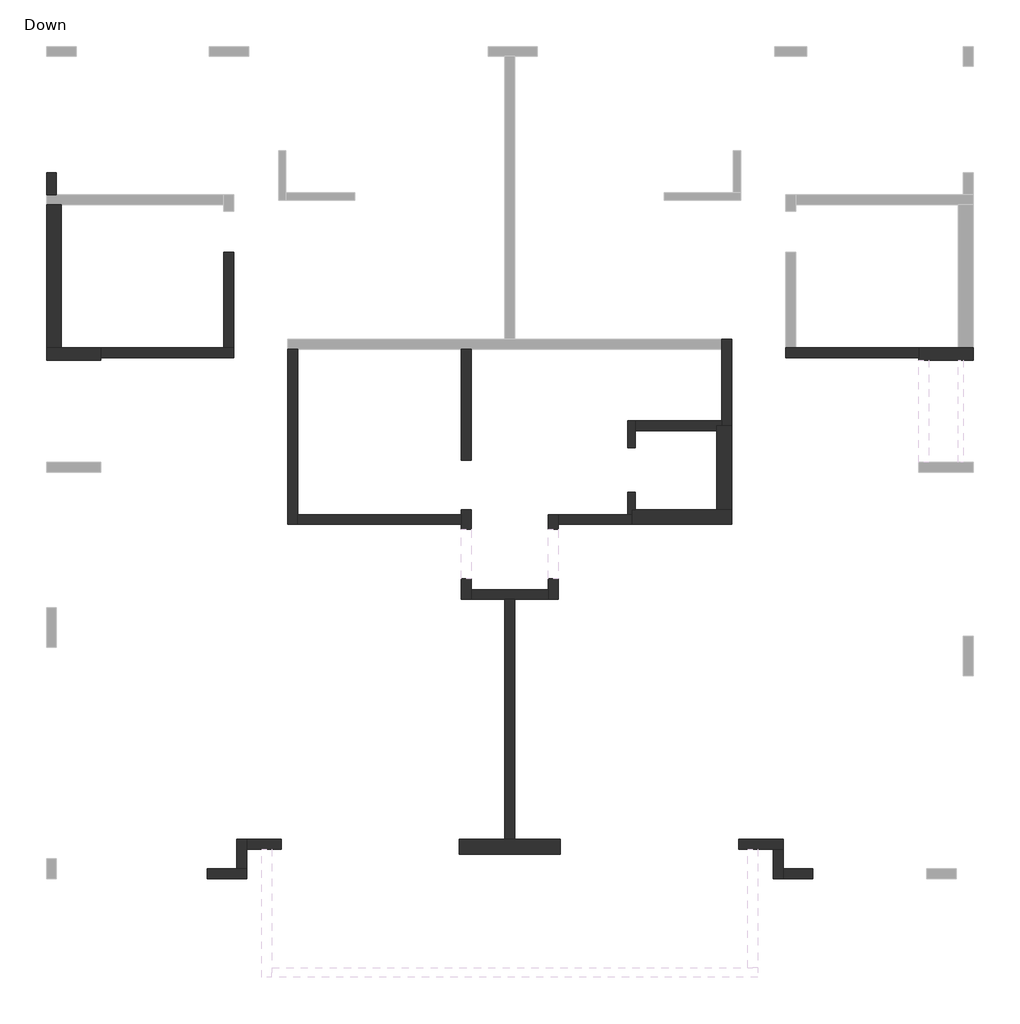
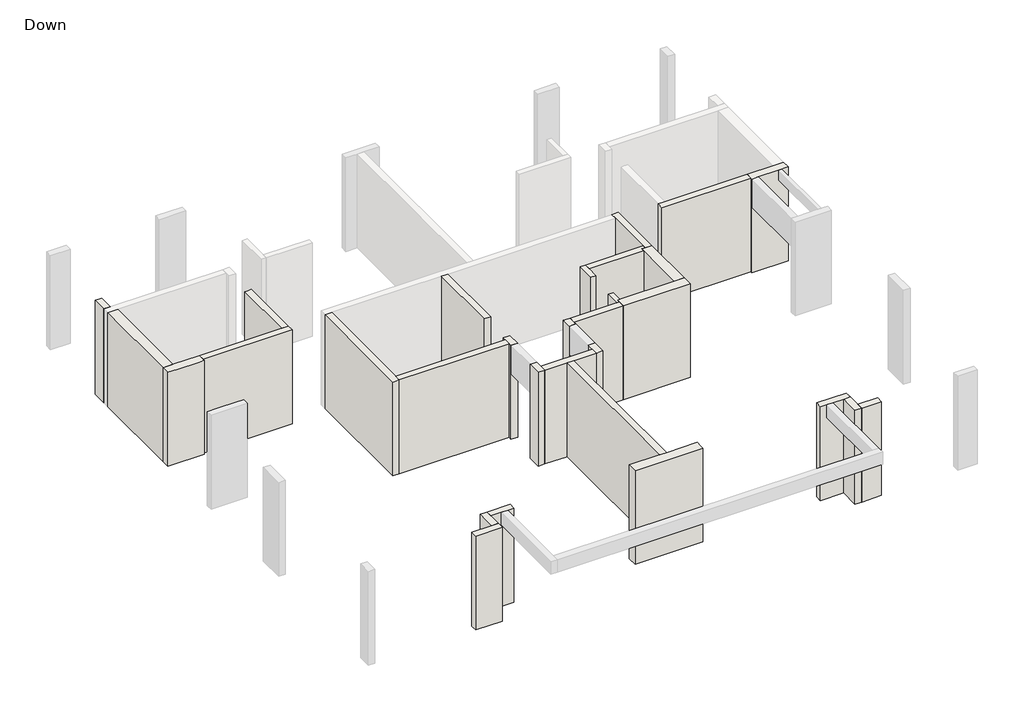
# One storey, part 1 of 2: 30 walls.
"""IFC4 building model written with IfcOpenShell, lengths in millimetres."""

from ifc_helpers import new_model, si_unit, origin, place, context, project, spatial, faceted_brep, element, save

model = new_model("IFC4")

# Units and contexts
model_context = context("Model", 3, world=origin())
ifc_project = project(units=[si_unit("LENGTHUNIT", "METRE", prefix="MILLI")], contexts=[model_context])

# Site, building, storey
site = spatial("IfcSite", under=ifc_project)
building = spatial("IfcBuilding", under=site)
storey = spatial("IfcBuildingStorey", under=building, Name="Down", Elevation=0.0)

# Walls
placement = place(None, origin())
element("IfcWall", 1, ObjectType="15", at=placement, inside=storey, context=model_context, shape_type="Brep", body=[
    faceted_brep([(-36032.8992549, 30554.4375606, 0.0), (-36032.8992549, 30005.16433, 0.0), (-36032.8992549, 30005.16433, 2780.0), (-36032.8992549, 30005.16433, 3000.0), (-36032.8992549, 30554.4375606, 3000.0), (-36032.8992549, 30554.4375606, 2780.0), (-35882.8992549, 30554.4375606, 0.0), (-35882.8992549, 30554.4375606, 3000.0), (-35882.8992549, 30354.4375606, 3000.0), (-35882.8992549, 30005.16433, 3000.0), (-35882.8992549, 30005.16433, 2780.0), (-35882.8992549, 30005.16433, 0.0), (-35882.8992549, 30354.4375606, 0.0)], [[[0, 1, 2, 3, 4, 5]], [[6, 7, 8, 9, 10, 11, 12]], [[1, 0, 6, 12, 11]], [[3, 2, 1, 11, 10, 9]], [[4, 3, 9, 8, 7]], [[0, 5, 4, 7, 6]]]),
])
element("IfcWall", 2, ObjectType="15", at=placement, inside=storey, context=model_context, shape_type="Brep", body=[
    faceted_brep([(-36032.8992549, 29103.4696053, 0.0), (-36032.8992549, 28654.7268324, 0.0), (-36032.8992549, 28654.7268324, 2780.0), (-36032.8992549, 28654.7268324, 3000.0), (-36032.8992549, 29103.4696053, 3000.0), (-36032.8992549, 29103.4696053, 2780.0), (-35882.8992549, 29103.4696053, 0.0), (-35882.8992549, 29103.4696053, 2780.0), (-35882.8992549, 29103.4696053, 3000.0), (-35882.8992549, 28754.7268324, 3000.0), (-35882.8992549, 28754.7268324, 0.0), (-35957.8992549, 28754.7268324, 0.0), (-35957.8992549, 28654.7268324, 0.0), (-35957.8992549, 28654.7268324, 3000.0), (-35957.8992549, 28754.7268324, 3000.0)], [[[0, 1, 2, 3, 4, 5]], [[6, 7, 8, 9, 10]], [[1, 0, 6, 10, 11, 12]], [[4, 3, 13, 14, 9, 8]], [[0, 5, 4, 8, 7, 6]], [[3, 2, 1, 12, 13]], [[12, 11, 14, 13]], [[11, 10, 9, 14]]]),
])
element("IfcWall", 3, ObjectType="20", at=placement, inside=storey, context=model_context, shape_type="Brep", body=[
    faceted_brep([(-38324.2014504, 22079.8085502, 0.0), (-38324.2014504, 26934.5299537, 0.0), (-38324.2014504, 26934.5299537, 2780.0), (-38324.2014504, 26934.5299537, 3000.0), (-38324.2014504, 22079.8085502, 3000.0), (-38324.2014504, 22079.8085502, 2780.0), (-38524.2014504, 22079.8085502, 0.0), (-38524.2014504, 22079.8085502, 2780.0), (-38524.2014504, 22079.8085502, 3000.0), (-38524.2014504, 26934.5299537, 3000.0), (-38524.2014504, 26934.5299537, 2780.0), (-38524.2014504, 26934.5299537, 0.0)], [[[0, 1, 2, 3, 4, 5]], [[6, 7, 8, 9, 10, 11]], [[1, 0, 6, 11]], [[4, 3, 9, 8]], [[3, 2, 1, 11, 10, 9]], [[0, 5, 4, 8, 7, 6]]]),
])
element("IfcWall", 4, ObjectType="20", at=placement, inside=storey, context=model_context, shape_type="Brep", body=[
    faceted_brep([(-39204.7173594, 26934.5299537, 0.0), (-38524.2014504, 26934.5299537, 0.0), (-38324.2014504, 26934.5299537, 0.0), (-37644.7021495, 26934.5299537, 0.0), (-37644.7021495, 26934.5299537, 3000.0), (-38324.2014504, 26934.5299537, 3000.0), (-38524.2014504, 26934.5299537, 3000.0), (-39204.7173594, 26934.5299537, 3000.0), (-39204.7173594, 27134.5299537, 0.0), (-39204.7173594, 27134.5299537, 2780.0), (-39204.7173594, 27134.5299537, 3000.0), (-37644.7021495, 27134.5299537, 3000.0), (-37644.7021495, 27134.5299537, 2780.0), (-37644.7021495, 27134.5299537, 0.0)], [[[0, 1, 2, 3, 4, 5, 6, 7]], [[8, 9, 10, 11, 12, 13]], [[3, 2, 1, 0, 8, 13]], [[7, 6, 5, 4, 11, 10]], [[4, 3, 13, 12, 11]], [[0, 7, 10, 9, 8]]]),
])
element("IfcWall", 5, ObjectType="20", at=placement, inside=storey, context=model_context, shape_type="Brep", body=[
    faceted_brep([(-37444.7021495, 26934.5299537, 0.0), (-37444.7021495, 27352.982888, 0.0), (-37444.7021495, 27352.982888, 2100.0), (-37444.7021495, 27352.982888, 3000.0), (-37444.7021495, 26934.5299537, 3000.0), (-37444.7021495, 26934.5299537, 2780.0), (-37644.7021495, 26934.5299537, 0.0), (-37644.7021495, 26934.5299537, 3000.0), (-37644.7021495, 27134.5299537, 3000.0), (-37644.7021495, 27352.982888, 3000.0), (-37644.7021495, 27352.982888, 2100.0), (-37644.7021495, 27352.982888, 0.0), (-37644.7021495, 27134.5299537, 0.0)], [[[0, 1, 2, 3, 4, 5]], [[6, 7, 8, 9, 10, 11, 12]], [[1, 0, 6, 12, 11]], [[3, 2, 1, 11, 10, 9]], [[4, 3, 9, 8, 7]], [[0, 5, 4, 7, 6]]]),
])
element("IfcWall", 6, ObjectType="20", at=placement, inside=storey, context=model_context, shape_type="Brep", body=[
    faceted_brep([(-39204.7173594, 26934.5299537, 0.0), (-39204.7173594, 27134.5299537, 0.0), (-39204.7173594, 27352.982888, 0.0), (-39204.7173594, 27352.982888, 2100.0), (-39204.7173594, 27352.982888, 3000.0), (-39204.7173594, 27134.5299537, 3000.0), (-39204.7173594, 26934.5299537, 3000.0), (-39404.7173594, 26934.5299537, 0.0), (-39404.7173594, 26934.5299537, 2780.0), (-39404.7173594, 26934.5299537, 3000.0), (-39404.7173594, 27352.982888, 3000.0), (-39404.7173594, 27352.982888, 2100.0), (-39404.7173594, 27352.982888, 0.0)], [[[0, 1, 2, 3, 4, 5, 6]], [[7, 8, 9, 10, 11, 12]], [[2, 1, 0, 7, 12]], [[4, 3, 2, 12, 11, 10]], [[6, 5, 4, 10, 9]], [[0, 6, 9, 8, 7]]]),
])
element("IfcWall", 7, ObjectType="20", at=placement, inside=storey, context=model_context, shape_type="Brep", body=[
    faceted_brep([(-37444.7021495, 28354.1914622, 0.0), (-37444.7021495, 28454.7268324, 0.0), (-37444.7021495, 28654.7268324, 0.0), (-37444.7021495, 28654.7268324, 3000.0), (-37444.7021495, 28454.7268324, 3000.0), (-37444.7021495, 28354.1914622, 3000.0), (-37444.7021495, 28354.1914622, 2100.0), (-37644.7021495, 28354.1914622, 0.0), (-37644.7021495, 28354.1914622, 2100.0), (-37644.7021495, 28354.1914622, 3000.0), (-37644.7021495, 28654.7268324, 3000.0), (-37644.7021495, 28654.7268324, 2780.0), (-37644.7021495, 28654.7268324, 0.0)], [[[0, 1, 2, 3, 4, 5, 6]], [[7, 8, 9, 10, 11, 12]], [[2, 1, 0, 7, 12]], [[5, 4, 3, 10, 9]], [[0, 6, 5, 9, 8, 7]], [[3, 2, 12, 11, 10]]]),
])
element("IfcWall", 8, ObjectType="20", at=placement, inside=storey, context=model_context, shape_type="Brep", body=[
    faceted_brep([(-37444.7021495, 28454.7268324, 0.0), (-35957.8992549, 28454.7268324, 0.0), (-35957.8992549, 28454.7268324, 3000.0), (-37444.7021495, 28454.7268324, 3000.0), (-37444.7021495, 28454.7268324, 2780.0), (-37444.7021495, 28654.7268324, 0.0), (-37444.7021495, 28654.7268324, 3000.0), (-36032.8992549, 28654.7268324, 3000.0), (-35957.8992549, 28654.7268324, 3000.0), (-35957.8992549, 28654.7268324, 0.0), (-36032.8992549, 28654.7268324, 0.0)], [[[0, 1, 2, 3, 4]], [[5, 6, 7, 8, 9, 10]], [[1, 0, 5, 10, 9]], [[2, 1, 9, 8]], [[3, 2, 8, 7, 6]], [[0, 4, 3, 6, 5]]]),
])
element("IfcWall", 9, ObjectType="20", at=placement, inside=storey, context=model_context, shape_type="Brep", body=[
    faceted_brep([(-33933.139307, 30454.4375606, 0.0), (-33933.139307, 32204.3938202, 0.0), (-33933.139307, 32204.3938202, 2780.0), (-33933.139307, 32204.3938202, 3000.0), (-33933.139307, 30454.4375606, 3000.0), (-34133.139307, 30454.4375606, 0.0), (-34133.139307, 30454.4375606, 3000.0), (-34133.139307, 30554.4375606, 3000.0), (-34133.139307, 32004.3938202, 3000.0), (-34133.139307, 32204.3938202, 3000.0), (-34133.139307, 32204.3938202, 0.0), (-34133.139307, 32004.3938202, 0.0), (-34133.139307, 30554.4375606, 0.0)], [[[0, 1, 2, 3, 4]], [[5, 6, 7, 8, 9, 10, 11, 12]], [[1, 0, 5, 12, 11, 10]], [[4, 3, 9, 8, 7, 6]], [[0, 4, 6, 5]], [[3, 2, 1, 10, 9]]]),
])
element("IfcWall", 10, ObjectType="20", at=placement, inside=storey, context=model_context, shape_type="Brep", body=[
    faceted_brep([(-42920.5336878, 32004.3938202, 0.0), (-42920.5336878, 28453.6610046, 0.0), (-42920.5336878, 28453.6610046, 2780.0), (-42920.5336878, 28453.6610046, 3000.0), (-42920.5336878, 32004.3938202, 3000.0), (-42720.5336878, 32004.3938202, 0.0), (-42720.5336878, 32004.3938202, 3000.0), (-42720.5336878, 28653.6610046, 3000.0), (-42720.5336878, 28453.6610046, 3000.0), (-42720.5336878, 28453.6610046, 0.0), (-42720.5336878, 28653.6610046, 0.0)], [[[0, 1, 2, 3, 4]], [[5, 6, 7, 8, 9, 10]], [[1, 0, 5, 10, 9]], [[4, 3, 8, 7, 6]], [[0, 4, 6, 5]], [[3, 2, 1, 9, 8]]]),
])
element("IfcWall", 11, ObjectType="20", at=placement, inside=storey, context=model_context, shape_type="Brep", body=[
    faceted_brep([(-42720.5336878, 28453.6610046, 0.0), (-39404.7173594, 28453.6610046, 0.0), (-39404.7173594, 28453.6610046, 2780.0), (-39404.7173594, 28453.6610046, 3000.0), (-42720.5336878, 28453.6610046, 3000.0), (-42720.5336878, 28653.6610046, 0.0), (-42720.5336878, 28653.6610046, 3000.0), (-40450.3660009, 28653.6610046, 3000.0), (-39404.7173594, 28653.6610046, 3000.0), (-39404.7173594, 28653.6610046, 2780.0), (-39404.7173594, 28653.6610046, 0.0)], [[[0, 1, 2, 3, 4]], [[5, 6, 7, 8, 9, 10]], [[1, 0, 5, 10]], [[4, 3, 8, 7, 6]], [[0, 4, 6, 5]], [[3, 2, 1, 10, 9, 8]]]),
])
element("IfcWall", 12, ObjectType="20", at=placement, inside=storey, context=model_context, shape_type="Brep", body=[
    faceted_brep([(-39404.7173594, 28754.2406819, 0.0), (-39404.7173594, 28653.6610046, 0.0), (-39404.7173594, 28453.6610046, 0.0), (-39404.7173594, 28354.1914622, 0.0), (-39404.7173594, 28354.1914622, 2100.0), (-39404.7173594, 28354.1914622, 3000.0), (-39404.7173594, 28453.6610046, 3000.0), (-39404.7173594, 28653.6610046, 3000.0), (-39404.7173594, 28754.2406819, 3000.0), (-39404.7173594, 28754.2406819, 2780.0), (-39204.7173594, 28754.2406819, 0.0), (-39204.7173594, 28754.2406819, 2780.0), (-39204.7173594, 28754.2406819, 3000.0), (-39204.7173594, 28354.1914622, 3000.0), (-39204.7173594, 28354.1914622, 2100.0), (-39204.7173594, 28354.1914622, 0.0)], [[[0, 1, 2, 3, 4, 5, 6, 7, 8, 9]], [[10, 11, 12, 13, 14, 15]], [[3, 2, 1, 0, 10, 15]], [[5, 4, 3, 15, 14, 13]], [[8, 7, 6, 5, 13, 12]], [[0, 9, 8, 12, 11, 10]]]),
])
element("IfcWall", 13, ObjectType="20", at=placement, inside=storey, context=model_context, shape_type="Brep", body=[
    faceted_brep([(-39204.7173594, 29753.278206, 0.0), (-39204.7173594, 32004.3938202, 0.0), (-39204.7173594, 32004.3938202, 2780.0), (-39204.7173594, 32004.3938202, 3000.0), (-39204.7173594, 29753.278206, 3000.0), (-39204.7173594, 29753.278206, 2780.0), (-39404.7173594, 29753.278206, 0.0), (-39404.7173594, 29753.278206, 2780.0), (-39404.7173594, 29753.278206, 3000.0), (-39404.7173594, 29837.9491617, 3000.0), (-39404.7173594, 32004.3938202, 3000.0), (-39404.7173594, 32004.3938202, 0.0)], [[[0, 1, 2, 3, 4, 5]], [[6, 7, 8, 9, 10, 11]], [[1, 0, 6, 11]], [[4, 3, 10, 9, 8]], [[0, 5, 4, 8, 7, 6]], [[3, 2, 1, 11, 10]]]),
])
element("IfcWall", 14, ObjectType="20", at=placement, inside=storey, context=model_context, shape_type="Brep", body=[
    faceted_brep([(-34133.139307, 30554.4375606, 0.0), (-35882.8992549, 30554.4375606, 0.0), (-35882.8992549, 30554.4375606, 3000.0), (-34133.139307, 30554.4375606, 3000.0), (-34133.139307, 30554.4375606, 2780.0), (-34233.139307, 30354.4375606, 0.0), (-34233.139307, 30354.4375606, 3000.0), (-35882.8992549, 30354.4375606, 3000.0), (-35882.8992549, 30354.4375606, 0.0), (-34133.139307, 30454.4375606, 0.0), (-34233.139307, 30454.4375606, 0.0), (-34233.139307, 30454.4375606, 3000.0), (-34133.139307, 30454.4375606, 3000.0)], [[[0, 1, 2, 3, 4]], [[5, 6, 7, 8]], [[1, 0, 9, 10, 5, 8]], [[3, 2, 7, 6, 11, 12]], [[0, 4, 3, 12, 9]], [[12, 11, 10, 9]], [[11, 6, 5, 10]], [[2, 1, 8, 7]]]),
])
element("IfcWall", 15, ObjectType="20", at=placement, inside=storey, context=model_context, shape_type="Brep", body=[
    faceted_brep([(-30144.302346, 32030.84273, 0.0), (-32634.5879334, 32030.84273, 0.0), (-32834.5879334, 32030.84273, 0.0), (-32834.5879334, 32030.84273, 3000.0), (-32634.5879334, 32030.84273, 3000.0), (-30144.302346, 32030.84273, 3000.0), (-30144.302346, 31830.84273, 0.0), (-30144.302346, 31830.84273, 2780.0), (-30144.302346, 31830.84273, 3000.0), (-32834.5879334, 31830.84273, 3000.0), (-32834.5879334, 31830.84273, 2780.0), (-32834.5879334, 31830.84273, 0.0)], [[[0, 1, 2, 3, 4, 5]], [[6, 7, 8, 9, 10, 11]], [[2, 1, 0, 6, 11]], [[5, 4, 3, 9, 8]], [[0, 5, 8, 7, 6]], [[3, 2, 11, 10, 9]]]),
])
element("IfcWall", 16, ObjectType="20", at=placement, inside=storey, context=model_context, shape_type="Brep", body=[
    faceted_brep([(-47805.7017527, 35580.4654108, 0.0), (-47805.7017527, 35129.640202, 0.0), (-47805.7017527, 35129.640202, 3000.0), (-47805.7017527, 35580.4654108, 3000.0), (-47805.7017527, 35580.4654108, 2780.0), (-47605.7017527, 35580.4654108, 0.0), (-47605.7017527, 35580.4654108, 2780.0), (-47605.7017527, 35580.4654108, 3000.0), (-47605.7017527, 35129.640202, 3000.0), (-47605.7017527, 35129.640202, 2780.0), (-47605.7017527, 35129.640202, 0.0)], [[[0, 1, 2, 3, 4]], [[5, 6, 7, 8, 9, 10]], [[1, 0, 5, 10]], [[3, 2, 8, 7]], [[0, 4, 3, 7, 6, 5]], [[2, 1, 10, 9, 8]]]),
])
element("IfcWall", 17, ObjectType="20", at=placement, inside=storey, context=model_context, shape_type="Brep", body=[
    faceted_brep([(-46705.7952795, 31830.84273, 0.0), (-44015.8481835, 31830.84273, 0.0), (-44015.8481835, 31830.84273, 2780.0), (-44015.8481835, 31830.84273, 3000.0), (-46705.7952795, 31830.84273, 3000.0), (-46705.7952795, 31830.84273, 2780.0), (-46705.7952795, 32030.84273, 0.0), (-46705.7952795, 32030.84273, 3000.0), (-44215.8481835, 32030.84273, 3000.0), (-44015.8481835, 32030.84273, 3000.0), (-44015.8481835, 32030.84273, 0.0), (-44215.8481835, 32030.84273, 0.0)], [[[0, 1, 2, 3, 4, 5]], [[6, 7, 8, 9, 10, 11]], [[1, 0, 6, 11, 10]], [[4, 3, 9, 8, 7]], [[0, 5, 4, 7, 6]], [[3, 2, 1, 10, 9]]]),
])
element("IfcWall", 18, ObjectType="20", at=placement, inside=storey, context=model_context, shape_type="Brep", body=[
    faceted_brep([(-44015.8481835, 32030.84273, 0.0), (-44015.8481835, 33965.4699454, 0.0), (-44015.8481835, 33965.4699454, 2780.0), (-44015.8481835, 33965.4699454, 3000.0), (-44015.8481835, 32030.84273, 3000.0), (-44215.8481835, 32030.84273, 0.0), (-44215.8481835, 32030.84273, 2780.0), (-44215.8481835, 32030.84273, 3000.0), (-44215.8481835, 33965.4699454, 3000.0), (-44215.8481835, 33965.4699454, 2780.0), (-44215.8481835, 33965.4699454, 0.0), (-44113.8149674, 33965.4699454, 3000.0)], [[[0, 1, 2, 3, 4]], [[5, 6, 7, 8, 9, 10]], [[1, 0, 5, 10]], [[3, 2, 1, 10, 9, 8, 11]], [[4, 3, 11, 8, 7]], [[0, 4, 7, 6, 5]]]),
])
element("IfcWall", 19, ObjectType="20", at=placement, inside=storey, context=model_context, shape_type="Brep", body=[
    faceted_brep([(-33786.4740574, 21880.2897882, 0.0), (-33086.4740574, 21880.2897882, 0.0), (-32886.4740574, 21880.2897882, 0.0), (-32886.4740574, 21880.2897882, 3000.0), (-33086.4740574, 21880.2897882, 3000.0), (-33405.0891993, 21880.2897882, 3000.0), (-33605.0891993, 21880.2897882, 3000.0), (-33786.4740574, 21880.2897882, 3000.0), (-33786.4740574, 21880.2897882, 2780.0), (-33786.4740574, 22080.2897882, 0.0), (-33786.4740574, 22080.2897882, 2780.0), (-33786.4740574, 22080.2897882, 3000.0), (-32886.4740574, 22080.2897882, 3000.0), (-32886.4740574, 22080.2897882, 2780.0), (-32886.4740574, 22080.2897882, 0.0)], [[[0, 1, 2, 3, 4, 5, 6, 7, 8]], [[9, 10, 11, 12, 13, 14]], [[2, 1, 0, 9, 14]], [[7, 6, 5, 4, 3, 12, 11]], [[0, 8, 7, 11, 10, 9]], [[3, 2, 14, 13, 12]]]),
])
element("IfcWall", 20, ObjectType="20", at=placement, inside=storey, context=model_context, shape_type="Brep", body=[
    faceted_brep([(-33086.4740574, 21880.2897882, 0.0), (-33086.4740574, 21280.2897882, 0.0), (-33086.4740574, 21280.2897882, 3000.0), (-33086.4740574, 21880.2897882, 3000.0), (-32886.4740574, 21880.2897882, 0.0), (-32886.4740574, 21880.2897882, 3000.0), (-32886.4740574, 21480.2897882, 3000.0), (-32886.4740574, 21280.2897882, 3000.0), (-32886.4740574, 21280.2897882, 0.0), (-32886.4740574, 21480.2897882, 0.0)], [[[0, 1, 2, 3]], [[4, 5, 6, 7, 8, 9]], [[1, 0, 4, 9, 8]], [[3, 2, 7, 6, 5]], [[0, 3, 5, 4]], [[2, 1, 8, 7]]]),
])
element("IfcWall", 21, ObjectType="20", at=placement, inside=storey, context=model_context, shape_type="Brep", body=[
    faceted_brep([(-32886.4740574, 21280.2897882, 0.0), (-32286.4740574, 21280.2897882, 0.0), (-32286.4740574, 21280.2897882, 2780.0), (-32286.4740574, 21280.2897882, 3000.0), (-32886.4740574, 21280.2897882, 3000.0), (-32886.4740574, 21480.2897882, 0.0), (-32886.4740574, 21480.2897882, 2780.0), (-32886.4740574, 21480.2897882, 3000.0), (-32286.4740574, 21480.2897882, 3000.0), (-32286.4740574, 21480.2897882, 2780.0), (-32286.4740574, 21480.2897882, 0.0)], [[[0, 1, 2, 3, 4]], [[5, 6, 7, 8, 9, 10]], [[1, 0, 5, 10]], [[3, 2, 1, 10, 9, 8]], [[4, 3, 8, 7]], [[0, 4, 7, 6, 5]]]),
])
element("IfcWall", 22, ObjectType="20", at=placement, inside=storey, context=model_context, shape_type="Brep", body=[
    faceted_brep([(-44556.7079689, 21280.2897882, 0.0), (-43756.7079689, 21280.2897882, 0.0), (-43756.7079689, 21280.2897882, 3000.0), (-44556.7079689, 21280.2897882, 3000.0), (-44556.7079689, 21280.2897882, 2780.0), (-44556.7079689, 21480.2897882, 0.0), (-44556.7079689, 21480.2897882, 2780.0), (-44556.7079689, 21480.2897882, 3000.0), (-43956.7079689, 21480.2897882, 3000.0), (-43756.7079689, 21480.2897882, 3000.0), (-43756.7079689, 21480.2897882, 0.0), (-43956.7079689, 21480.2897882, 0.0)], [[[0, 1, 2, 3, 4]], [[5, 6, 7, 8, 9, 10, 11]], [[1, 0, 5, 11, 10]], [[3, 2, 9, 8, 7]], [[0, 4, 3, 7, 6, 5]], [[2, 1, 10, 9]]]),
])
element("IfcWall", 23, ObjectType="20", at=placement, inside=storey, context=model_context, shape_type="Brep", body=[
    faceted_brep([(-43756.7079689, 21480.2897882, 0.0), (-43756.7079689, 21880.2897882, 0.0), (-43756.7079689, 22080.2897882, 0.0), (-43756.7079689, 22080.2897882, 3000.0), (-43756.7079689, 21880.2897882, 3000.0), (-43756.7079689, 21480.2897882, 3000.0), (-43956.7079689, 21480.2897882, 0.0), (-43956.7079689, 21480.2897882, 2780.0), (-43956.7079689, 21480.2897882, 3000.0), (-43956.7079689, 22080.2897882, 3000.0), (-43956.7079689, 22080.2897882, 2780.0), (-43956.7079689, 22080.2897882, 0.0)], [[[0, 1, 2, 3, 4, 5]], [[6, 7, 8, 9, 10, 11]], [[2, 1, 0, 6, 11]], [[5, 4, 3, 9, 8]], [[0, 5, 8, 7, 6]], [[3, 2, 11, 10, 9]]]),
])
element("IfcWall", 24, ObjectType="20", at=placement, inside=storey, context=model_context, shape_type="Brep", body=[
    faceted_brep([(-43756.7079689, 21880.2897882, 0.0), (-43056.7079689, 21880.2897882, 0.0), (-43056.7079689, 21880.2897882, 2780.0), (-43056.7079689, 21880.2897882, 3000.0), (-43243.3137014, 21880.2897882, 3000.0), (-43443.3137014, 21880.2897882, 3000.0), (-43756.7079689, 21880.2897882, 3000.0), (-43756.7079689, 22080.2897882, 0.0), (-43756.7079689, 22080.2897882, 3000.0), (-43056.7079689, 22080.2897882, 3000.0), (-43056.7079689, 22080.2897882, 2780.0), (-43056.7079689, 22080.2897882, 0.0)], [[[0, 1, 2, 3, 4, 5, 6]], [[7, 8, 9, 10, 11]], [[1, 0, 7, 11]], [[3, 2, 1, 11, 10, 9]], [[6, 5, 4, 3, 9, 8]], [[0, 6, 8, 7]]]),
])
element("IfcWall", 25, ObjectType="25", at=placement, inside=storey, context=model_context, shape_type="Brep", body=[
    faceted_brep([(-29044.7343642, 32030.84273, 0.0), (-29344.7343642, 32030.84273, 0.0), (-30144.302346, 32030.84273, 0.0), (-30144.302346, 32030.84273, 3000.0), (-29344.7343642, 32030.84273, 3000.0), (-29044.7343642, 32030.84273, 3000.0), (-29044.7343642, 31780.84273, 0.0), (-29044.7343642, 31780.84273, 3000.0), (-29340.5251854, 31780.84273, 3000.0), (-29944.302346, 31780.84273, 3000.0), (-30144.302346, 31780.84273, 3000.0), (-30144.302346, 31780.84273, 0.0), (-30144.302346, 31830.84273, 0.0), (-30144.302346, 31830.84273, 3000.0)], [[[0, 1, 2, 3, 4, 5]], [[6, 7, 8, 9, 10, 11]], [[2, 1, 0, 6, 11, 12]], [[3, 2, 12, 11, 10, 13]], [[5, 4, 3, 13, 10, 9, 8, 7]], [[0, 5, 7, 6]]]),
])
element("IfcWall", 26, ObjectType="25", at=placement, inside=storey, context=model_context, shape_type="Brep", body=[
    faceted_brep([(-47805.7017527, 31780.84273, 0.0), (-46705.7952795, 31780.84273, 0.0), (-46705.7952795, 31780.84273, 3000.0), (-46905.7952795, 31780.84273, 3000.0), (-47505.2156022, 31780.84273, 3000.0), (-47805.7017527, 31780.84273, 3000.0), (-47805.7017527, 32030.84273, 0.0), (-47805.7017527, 32030.84273, 3000.0), (-47505.7017527, 32030.84273, 3000.0), (-46705.7952795, 32030.84273, 3000.0), (-46705.7952795, 32030.84273, 0.0), (-47505.7017527, 32030.84273, 0.0), (-46705.7952795, 31830.84273, 0.0), (-46705.7952795, 31830.84273, 3000.0)], [[[0, 1, 2, 3, 4, 5]], [[6, 7, 8, 9, 10, 11]], [[1, 0, 6, 11, 10, 12]], [[2, 1, 12, 10, 9, 13]], [[5, 4, 3, 2, 13, 9, 8, 7]], [[0, 5, 7, 6]]]),
])
element("IfcWall", 27, ObjectType="30", at=placement, inside=storey, context=model_context, shape_type="Brep", body=[
    faceted_brep([(-39449.2017338, 21779.8085502, 0.0), (-37400.2620822, 21779.8085502, 0.0), (-37400.2620822, 21779.8085502, 2540.0), (-37400.2620822, 21779.8085502, 2800.0), (-37400.2620822, 21779.8085502, 3000.0), (-39449.2017338, 21779.8085502, 3000.0), (-39449.2017338, 21779.8085502, 2800.0), (-39449.2017338, 21779.8085502, 2540.0), (-39449.2017338, 22079.8085502, 0.0), (-39449.2017338, 22079.8085502, 2780.0), (-39449.2017338, 22079.8085502, 3000.0), (-38524.2014504, 22079.8085502, 3000.0), (-38324.2014504, 22079.8085502, 3000.0), (-37400.2620822, 22079.8085502, 3000.0), (-37400.2620822, 22079.8085502, 2780.0), (-37400.2620822, 22079.8085502, 0.0), (-38324.2014504, 22079.8085502, 0.0), (-38524.2014504, 22079.8085502, 0.0), (-37400.2620822, 21880.2897882, 3000.0), (-39449.2017338, 21880.2897882, 3000.0)], [[[0, 1, 2, 3, 4, 5, 6, 7]], [[8, 9, 10, 11, 12, 13, 14, 15, 16, 17]], [[1, 0, 8, 17, 16, 15]], [[4, 3, 2, 1, 15, 14, 13, 18]], [[5, 4, 18, 13, 12, 11, 10, 19]], [[0, 7, 6, 5, 19, 10, 9, 8]]]),
])
element("IfcWall", 28, ObjectType="30", at=placement, inside=storey, context=model_context, shape_type="Brep", body=[
    faceted_brep([(-33933.139307, 28754.7268324, 0.0), (-34233.139307, 28754.7268324, 0.0), (-35882.8992549, 28754.7268324, 0.0), (-35957.8992549, 28754.7268324, 0.0), (-35957.8992549, 28754.7268324, 3000.0), (-35882.8992549, 28754.7268324, 3000.0), (-34233.139307, 28754.7268324, 3000.0), (-33933.139307, 28754.7268324, 3000.0), (-33933.139307, 28454.7268324, 0.0), (-33933.139307, 28454.7268324, 2780.0), (-33933.139307, 28454.7268324, 3000.0), (-35957.8992549, 28454.7268324, 3000.0), (-35957.8992549, 28454.7268324, 0.0), (-35957.8992549, 28654.7268324, 0.0), (-35957.8992549, 28654.7268324, 3000.0)], [[[0, 1, 2, 3, 4, 5, 6, 7]], [[8, 9, 10, 11, 12]], [[3, 2, 1, 0, 8, 12, 13]], [[4, 3, 13, 12, 11, 14]], [[7, 6, 5, 4, 14, 11, 10]], [[0, 7, 10, 9, 8]]]),
])
element("IfcWall", 29, ObjectType="30", at=placement, inside=storey, context=model_context, shape_type="Brep", body=[
    faceted_brep([(-33933.139307, 28754.7268324, 0.0), (-33933.139307, 30454.4375606, 0.0), (-33933.139307, 30454.4375606, 3000.0), (-33933.139307, 28754.7268324, 3000.0), (-34233.139307, 28754.7268324, 0.0), (-34233.139307, 28754.7268324, 3000.0), (-34233.139307, 30354.4375606, 3000.0), (-34233.139307, 30454.4375606, 3000.0), (-34233.139307, 30454.4375606, 0.0), (-34233.139307, 30354.4375606, 0.0), (-34133.139307, 30454.4375606, 0.0), (-34133.139307, 30454.4375606, 3000.0)], [[[0, 1, 2, 3]], [[4, 5, 6, 7, 8, 9]], [[1, 0, 4, 9, 8, 10]], [[2, 1, 10, 8, 7, 11]], [[3, 2, 11, 7, 6, 5]], [[0, 3, 5, 4]]]),
])
element("IfcWall", 30, ObjectType="30", at=placement, inside=storey, context=model_context, shape_type="Brep", body=[
    faceted_brep([(-47805.7017527, 34929.640202, 0.0), (-47805.7017527, 32030.84273, 0.0), (-47805.7017527, 32030.84273, 3000.0), (-47805.7017527, 34929.640202, 3000.0), (-47505.7017527, 34929.640202, 0.0), (-47505.7017527, 34929.640202, 2780.0), (-47505.7017527, 34929.640202, 3000.0), (-47505.7017527, 32030.84273, 3000.0), (-47505.7017527, 32030.84273, 2780.0), (-47505.7017527, 32030.84273, 0.0)], [[[0, 1, 2, 3]], [[4, 5, 6, 7, 8, 9]], [[1, 0, 4, 9]], [[3, 2, 7, 6]], [[2, 1, 9, 8, 7]], [[0, 3, 6, 5, 4]]]),
])

save(model, "model.ifc")

# Revit data of these elements
# Project information
#   Project Issue Date = "Issue Date"
#   Project Status = "Project Status"
#   Client Name = "לקוח"
#   Project Address = "Enter address here"
#   Project Name = "Project 009"
#   Project Number = "מספר פרויקט"
# Type "15"
#   Layers, outside or top first: 15 cm "Concrete" (function 1)
# Type "20"
#   Layers, outside or top first: 20 cm "Concrete" (function 1)
# Type "25"
#   Layers, outside or top first: 25 cm "Concrete" (function 1)
# Type "30"
#   Layers, outside or top first: 30 cm "Concrete" (function 1)
# Element 1 (IfcWall, "15")
#   Comments = ""
#   Mark = "W5"
#   SOFiSTiK_EdgeZones = "W5"
#   SOFiSTiK_AMG_Comments = ""
#   Top Offset = 0 cm
#   Base Offset = 0 cm
#   wall height = 300 cm
#   SOFiSTiK_AMG_Scheduled = yes
#   SOFiSTiK_AMG_Adjusted = yes
#   Phase Created = New Construction
#   Base Constraint = Down
#   Top Constraint = Typical Floor
#   Materials on its faces: "Concrete"
# Element 2 (IfcWall, "15")
#   Comments = ""
#   Mark = "W6"
#   SOFiSTiK_EdgeZones = "W6"
#   SOFiSTiK_AMG_Comments = ""
#   Top Offset = 0 cm
#   Base Offset = 0 cm
#   wall height = 300 cm
#   SOFiSTiK_AMG_Scheduled = yes
#   SOFiSTiK_AMG_Adjusted = yes
#   Phase Created = New Construction
#   Base Constraint = Down
#   Top Constraint = Typical Floor
#   Materials on its faces: "Concrete"
# Element 3 (IfcWall, "20")
#   Comments = ""
#   Mark = "W12"
#   SOFiSTiK_EdgeZones = "W12"
#   SOFiSTiK_AMG_Comments = ""
#   Top Offset = 0 cm
#   Base Offset = 0 cm
#   wall height = 300 cm
#   SOFiSTiK_AMG_Scheduled = yes
#   SOFiSTiK_AMG_Adjusted = yes
#   Phase Created = New Construction
#   Base Constraint = Down
#   Top Constraint = Typical Floor
#   Materials on its faces: "Concrete"
# Element 4 (IfcWall, "20")
#   Comments = ""
#   Mark = "W13"
#   SOFiSTiK_EdgeZones = "W13"
#   SOFiSTiK_AMG_Comments = ""
#   Top Offset = 0 cm
#   Base Offset = 0 cm
#   wall height = 300 cm
#   SOFiSTiK_AMG_Scheduled = yes
#   SOFiSTiK_AMG_Adjusted = yes
#   Phase Created = New Construction
#   Base Constraint = Down
#   Top Constraint = Typical Floor
#   Materials on its faces: "Concrete"
# Element 5 (IfcWall, "20")
#   Comments = ""
#   Mark = "W14"
#   SOFiSTiK_EdgeZones = "W14"
#   SOFiSTiK_AMG_Comments = ""
#   Top Offset = 0 cm
#   Base Offset = 0 cm
#   wall height = 300 cm
#   SOFiSTiK_AMG_Scheduled = yes
#   SOFiSTiK_AMG_Adjusted = yes
#   Phase Created = New Construction
#   Base Constraint = Down
#   Top Constraint = Typical Floor
#   Materials on its faces: "Concrete"
# Element 6 (IfcWall, "20")
#   Comments = ""
#   Mark = "W15"
#   SOFiSTiK_EdgeZones = "W15"
#   SOFiSTiK_AMG_Comments = ""
#   Top Offset = 0 cm
#   Base Offset = 0 cm
#   wall height = 300 cm
#   SOFiSTiK_AMG_Scheduled = yes
#   SOFiSTiK_AMG_Adjusted = yes
#   Phase Created = New Construction
#   Base Constraint = Down
#   Top Constraint = Typical Floor
#   Materials on its faces: "Concrete"
# Element 7 (IfcWall, "20")
#   Comments = ""
#   Mark = "W16"
#   SOFiSTiK_EdgeZones = "W16"
#   SOFiSTiK_AMG_Comments = ""
#   Top Offset = 0 cm
#   Base Offset = 0 cm
#   wall height = 300 cm
#   SOFiSTiK_AMG_Scheduled = yes
#   SOFiSTiK_AMG_Adjusted = yes
#   Phase Created = New Construction
#   Base Constraint = Down
#   Top Constraint = Typical Floor
#   Materials on its faces: "Concrete"
# Element 8 (IfcWall, "20")
#   Comments = ""
#   Mark = "W17"
#   SOFiSTiK_EdgeZones = "W17"
#   SOFiSTiK_AMG_Comments = ""
#   Top Offset = 0 cm
#   Base Offset = 0 cm
#   wall height = 300 cm
#   SOFiSTiK_AMG_Scheduled = yes
#   SOFiSTiK_AMG_Adjusted = yes
#   Phase Created = New Construction
#   Base Constraint = Down
#   Top Constraint = Typical Floor
#   Materials on its faces: "Concrete"
# Element 9 (IfcWall, "20")
#   Comments = ""
#   Mark = "W18"
#   SOFiSTiK_EdgeZones = "W18"
#   SOFiSTiK_AMG_Comments = ""
#   Top Offset = 0 cm
#   Base Offset = 0 cm
#   wall height = 300 cm
#   SOFiSTiK_AMG_Scheduled = yes
#   SOFiSTiK_AMG_Adjusted = yes
#   Phase Created = New Construction
#   Base Constraint = Down
#   Top Constraint = Typical Floor
#   Materials on its faces: "Concrete"
# Element 10 (IfcWall, "20")
#   Comments = ""
#   Mark = "W20"
#   SOFiSTiK_EdgeZones = "W20"
#   SOFiSTiK_AMG_Comments = ""
#   Top Offset = 0 cm
#   Base Offset = 0 cm
#   wall height = 300 cm
#   SOFiSTiK_AMG_Scheduled = yes
#   SOFiSTiK_AMG_Adjusted = yes
#   Phase Created = New Construction
#   Base Constraint = Down
#   Top Constraint = Typical Floor
#   Materials on its faces: "Concrete"
# Element 11 (IfcWall, "20")
#   Comments = ""
#   Mark = "W21"
#   SOFiSTiK_EdgeZones = "W21"
#   SOFiSTiK_AMG_Comments = ""
#   Top Offset = 0 cm
#   Base Offset = 0 cm
#   wall height = 300 cm
#   SOFiSTiK_AMG_Scheduled = yes
#   SOFiSTiK_AMG_Adjusted = yes
#   Phase Created = New Construction
#   Base Constraint = Down
#   Top Constraint = Typical Floor
#   Materials on its faces: "Concrete"
# Element 12 (IfcWall, "20")
#   Comments = ""
#   Mark = "W22"
#   SOFiSTiK_EdgeZones = "W22"
#   SOFiSTiK_AMG_Comments = ""
#   Top Offset = 0 cm
#   Base Offset = 0 cm
#   wall height = 300 cm
#   SOFiSTiK_AMG_Scheduled = yes
#   SOFiSTiK_AMG_Adjusted = yes
#   Phase Created = New Construction
#   Base Constraint = Down
#   Top Constraint = Typical Floor
#   Materials on its faces: "Concrete"
# Element 13 (IfcWall, "20")
#   Comments = ""
#   Mark = "W23"
#   SOFiSTiK_EdgeZones = "W23"
#   SOFiSTiK_AMG_Comments = ""
#   Top Offset = 0 cm
#   Base Offset = 0 cm
#   wall height = 300 cm
#   SOFiSTiK_AMG_Scheduled = yes
#   SOFiSTiK_AMG_Adjusted = yes
#   Phase Created = New Construction
#   Base Constraint = Down
#   Top Constraint = Typical Floor
#   Materials on its faces: "Concrete"
# Element 14 (IfcWall, "20")
#   Comments = ""
#   Mark = "W24"
#   SOFiSTiK_EdgeZones = "W24"
#   SOFiSTiK_AMG_Comments = ""
#   Top Offset = 0 cm
#   Base Offset = 0 cm
#   wall height = 300 cm
#   SOFiSTiK_AMG_Scheduled = yes
#   SOFiSTiK_AMG_Adjusted = yes
#   Phase Created = New Construction
#   Base Constraint = Down
#   Top Constraint = Typical Floor
#   Materials on its faces: "Concrete"
# Element 15 (IfcWall, "20")
#   Comments = ""
#   Mark = "W27"
#   SOFiSTiK_EdgeZones = "W27"
#   SOFiSTiK_AMG_Comments = ""
#   Top Offset = 0 cm
#   Base Offset = 0 cm
#   wall height = 300 cm
#   SOFiSTiK_AMG_Scheduled = yes
#   SOFiSTiK_AMG_Adjusted = yes
#   Phase Created = New Construction
#   Base Constraint = Down
#   Top Constraint = Typical Floor
#   Materials on its faces: "Concrete"
# Element 16 (IfcWall, "20")
#   Comments = ""
#   Mark = "W31"
#   SOFiSTiK_EdgeZones = "W31"
#   SOFiSTiK_AMG_Comments = ""
#   Top Offset = 0 cm
#   Base Offset = 0 cm
#   wall height = 300 cm
#   SOFiSTiK_AMG_Scheduled = yes
#   SOFiSTiK_AMG_Adjusted = yes
#   Phase Created = New Construction
#   Base Constraint = Down
#   Top Constraint = Typical Floor
#   Materials on its faces: "Concrete"
# Element 17 (IfcWall, "20")
#   Comments = ""
#   Mark = "W32"
#   SOFiSTiK_EdgeZones = "W32"
#   SOFiSTiK_AMG_Comments = ""
#   Top Offset = 0 cm
#   Base Offset = 0 cm
#   wall height = 300 cm
#   SOFiSTiK_AMG_Scheduled = yes
#   SOFiSTiK_AMG_Adjusted = yes
#   Phase Created = New Construction
#   Base Constraint = Down
#   Top Constraint = Typical Floor
#   Materials on its faces: "Concrete"
# Element 18 (IfcWall, "20")
#   Comments = ""
#   Mark = "W33"
#   SOFiSTiK_EdgeZones = "W33"
#   SOFiSTiK_AMG_Comments = ""
#   Top Offset = 0 cm
#   Base Offset = 0 cm
#   wall height = 300 cm
#   SOFiSTiK_AMG_Scheduled = yes
#   SOFiSTiK_AMG_Adjusted = yes
#   Phase Created = New Construction
#   Base Constraint = Down
#   Top Constraint = Typical Floor
#   Materials on its faces: "Concrete"
# Element 19 (IfcWall, "20")
#   Comments = ""
#   Mark = "W36"
#   SOFiSTiK_EdgeZones = "W36"
#   SOFiSTiK_AMG_Comments = ""
#   Top Offset = 0 cm
#   Base Offset = 0 cm
#   wall height = 300 cm
#   SOFiSTiK_AMG_Scheduled = yes
#   SOFiSTiK_AMG_Adjusted = yes
#   Phase Created = New Construction
#   Base Constraint = Down
#   Top Constraint = Typical Floor
#   Materials on its faces: "Concrete"
# Element 20 (IfcWall, "20")
#   Comments = ""
#   Mark = "W37"
#   SOFiSTiK_EdgeZones = "W37"
#   SOFiSTiK_AMG_Comments = ""
#   Top Offset = 0 cm
#   Base Offset = 0 cm
#   wall height = 300 cm
#   SOFiSTiK_AMG_Scheduled = yes
#   SOFiSTiK_AMG_Adjusted = yes
#   Phase Created = New Construction
#   Base Constraint = Down
#   Top Constraint = Typical Floor
#   Materials on its faces: "Concrete"
# Element 21 (IfcWall, "20")
#   Comments = ""
#   Mark = "W38"
#   SOFiSTiK_EdgeZones = "W38"
#   SOFiSTiK_AMG_Comments = ""
#   Top Offset = 0 cm
#   Base Offset = 0 cm
#   wall height = 300 cm
#   SOFiSTiK_AMG_Scheduled = yes
#   SOFiSTiK_AMG_Adjusted = yes
#   Phase Created = New Construction
#   Base Constraint = Down
#   Top Constraint = Typical Floor
#   Materials on its faces: "Concrete"
# Element 22 (IfcWall, "20")
#   Comments = ""
#   Mark = "W39"
#   SOFiSTiK_EdgeZones = "W39"
#   SOFiSTiK_AMG_Comments = ""
#   Top Offset = 0 cm
#   Base Offset = 0 cm
#   wall height = 300 cm
#   SOFiSTiK_AMG_Scheduled = yes
#   SOFiSTiK_AMG_Adjusted = yes
#   Phase Created = New Construction
#   Base Constraint = Down
#   Top Constraint = Typical Floor
#   Materials on its faces: "Concrete"
# Element 23 (IfcWall, "20")
#   Comments = ""
#   Mark = "W40"
#   SOFiSTiK_EdgeZones = "W40"
#   SOFiSTiK_AMG_Comments = ""
#   Top Offset = 0 cm
#   Base Offset = 0 cm
#   wall height = 300 cm
#   SOFiSTiK_AMG_Scheduled = yes
#   SOFiSTiK_AMG_Adjusted = yes
#   Phase Created = New Construction
#   Base Constraint = Down
#   Top Constraint = Typical Floor
#   Materials on its faces: "Concrete"
# Element 24 (IfcWall, "20")
#   Comments = ""
#   Mark = "W41"
#   SOFiSTiK_EdgeZones = "W41"
#   SOFiSTiK_AMG_Comments = ""
#   Top Offset = 0 cm
#   Base Offset = 0 cm
#   wall height = 300 cm
#   SOFiSTiK_AMG_Scheduled = yes
#   SOFiSTiK_AMG_Adjusted = yes
#   Phase Created = New Construction
#   Base Constraint = Down
#   Top Constraint = Typical Floor
#   Materials on its faces: "Concrete"
# Element 25 (IfcWall, "25")
#   Comments = ""
#   Mark = "W42"
#   SOFiSTiK_EdgeZones = "W42"
#   SOFiSTiK_AMG_Comments = ""
#   Top Offset = 0 cm
#   Base Offset = 0 cm
#   wall height = 300 cm
#   SOFiSTiK_AMG_Scheduled = yes
#   SOFiSTiK_AMG_Adjusted = yes
#   Phase Created = New Construction
#   Base Constraint = Down
#   Top Constraint = Typical Floor
#   Materials on its faces: "Concrete"
# Element 26 (IfcWall, "25")
#   Comments = ""
#   Mark = "W43"
#   SOFiSTiK_EdgeZones = "W43"
#   SOFiSTiK_AMG_Comments = ""
#   Top Offset = 0 cm
#   Base Offset = 0 cm
#   wall height = 300 cm
#   SOFiSTiK_AMG_Scheduled = yes
#   SOFiSTiK_AMG_Adjusted = yes
#   Phase Created = New Construction
#   Base Constraint = Down
#   Top Constraint = Typical Floor
#   Materials on its faces: "Concrete"
# Element 27 (IfcWall, "30")
#   Comments = ""
#   Mark = "W7"
#   SOFiSTiK_EdgeZones = "W7"
#   SOFiSTiK_AMG_Comments = ""
#   Top Offset = 0 cm
#   Base Offset = 0 cm
#   wall height = 300 cm
#   SOFiSTiK_AMG_Scheduled = yes
#   SOFiSTiK_AMG_Adjusted = yes
#   Phase Created = New Construction
#   Base Constraint = Down
#   Top Constraint = Typical Floor
#   Materials on its faces: "Concrete"
# Element 28 (IfcWall, "30")
#   Comments = ""
#   Mark = "W8"
#   SOFiSTiK_EdgeZones = "W8"
#   SOFiSTiK_AMG_Comments = ""
#   Top Offset = 0 cm
#   Base Offset = 0 cm
#   wall height = 300 cm
#   SOFiSTiK_AMG_Scheduled = yes
#   SOFiSTiK_AMG_Adjusted = yes
#   Phase Created = New Construction
#   Base Constraint = Down
#   Top Constraint = Typical Floor
#   Materials on its faces: "Concrete"
# Element 29 (IfcWall, "30")
#   Comments = ""
#   Mark = "W9"
#   SOFiSTiK_EdgeZones = "W9"
#   SOFiSTiK_AMG_Comments = ""
#   Top Offset = 0 cm
#   Base Offset = 0 cm
#   wall height = 300 cm
#   SOFiSTiK_AMG_Scheduled = yes
#   SOFiSTiK_AMG_Adjusted = yes
#   Phase Created = New Construction
#   Base Constraint = Down
#   Top Constraint = Typical Floor
#   Materials on its faces: "Concrete"
# Element 30 (IfcWall, "30")
#   Comments = ""
#   Mark = "W11"
#   SOFiSTiK_EdgeZones = "W11"
#   SOFiSTiK_AMG_Comments = ""
#   Top Offset = 0 cm
#   Base Offset = 0 cm
#   wall height = 300 cm
#   SOFiSTiK_AMG_Scheduled = yes
#   SOFiSTiK_AMG_Adjusted = yes
#   Phase Created = New Construction
#   Base Constraint = Down
#   Top Constraint = Typical Floor
#   Materials on its faces: "Concrete"
# Materials
#   "Concrete": class "Concrete", colour RGB 192 192 192, transparency 0, Keynote = "01000", Description = "Cast-in-place concrete", Cost = 0
